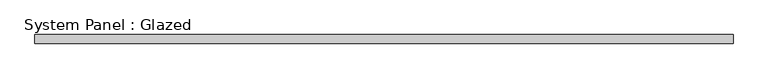
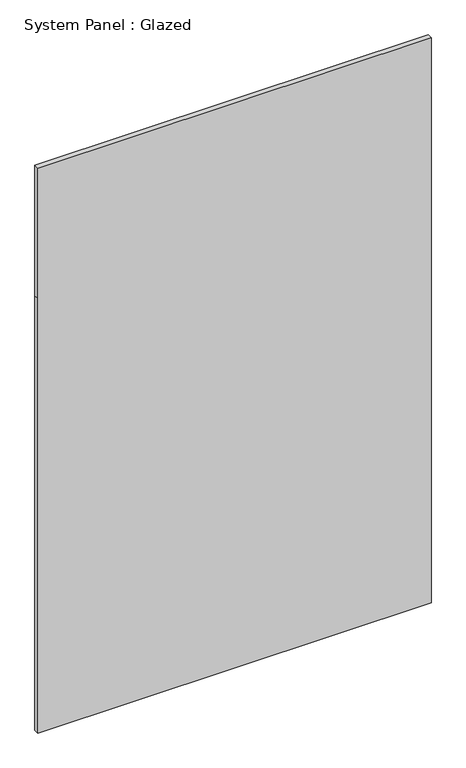
"""IFC4 building model written with IfcOpenShell, lengths in millimetres: plate geometry, System Panel : Glazed."""

from ifc_helpers import new_model, si_unit, frame, origin, place, context, project, spatial, polyline, outline, extrude, source, transform, mapped, element, save


def system_panel_glazed_5de2274e(model_context):
    return source(origin(), model_context, "Body", "SweptSolid", [
        extrude(outline(polyline([(0.0, -962.5000001), (0.0, 962.5000001), (2250.0, 962.5000001), (2925.0, 962.5000001), (2925.0, -962.5000001), (2250.0, -962.5000001), (0.0, -962.5000001)])), frame((0.0, 24.5, 0.0), z_axis=(0.0, 1.0, 0.0), x_axis=(0.0, 0.0, 1.0)), (0.0, 0.0, 1.0), 25.0),
    ])


if __name__ == "__main__":
    model = new_model("IFC4")
    model_context = context("Model", 3, world=origin())
    ifc_project = project(units=[si_unit("LENGTHUNIT", "METRE", prefix="MILLI")], contexts=[model_context])
    site = spatial("IfcSite", under=ifc_project)
    building = spatial("IfcBuilding", under=site)
    placement = place(None, origin())
    system_panel_glazed_shape = system_panel_glazed_5de2274e(model_context)
    element("IfcPlate", 1, ObjectType="System Panel : Glazed", at=placement, inside=building, context=model_context, shape_type="MappedRepresentation", body=[
        mapped(system_panel_glazed_shape, transform((0.0, 0.0, 0.0), x_axis=(1.0, 0.0, 0.0), y_axis=(0.0, 1.0, 0.0), z_axis=(0.0, 0.0, 1.0))),
    ])
    save(model, "model.ifc")

# Revit data of these elements
# Element 1 (IfcPlate, "System Panel : Glazed")
#   Materials on its faces: "Glass"
# Materials
#   "Glass": class "Glass", colour RGB 0 128 192, transparency 0.9
